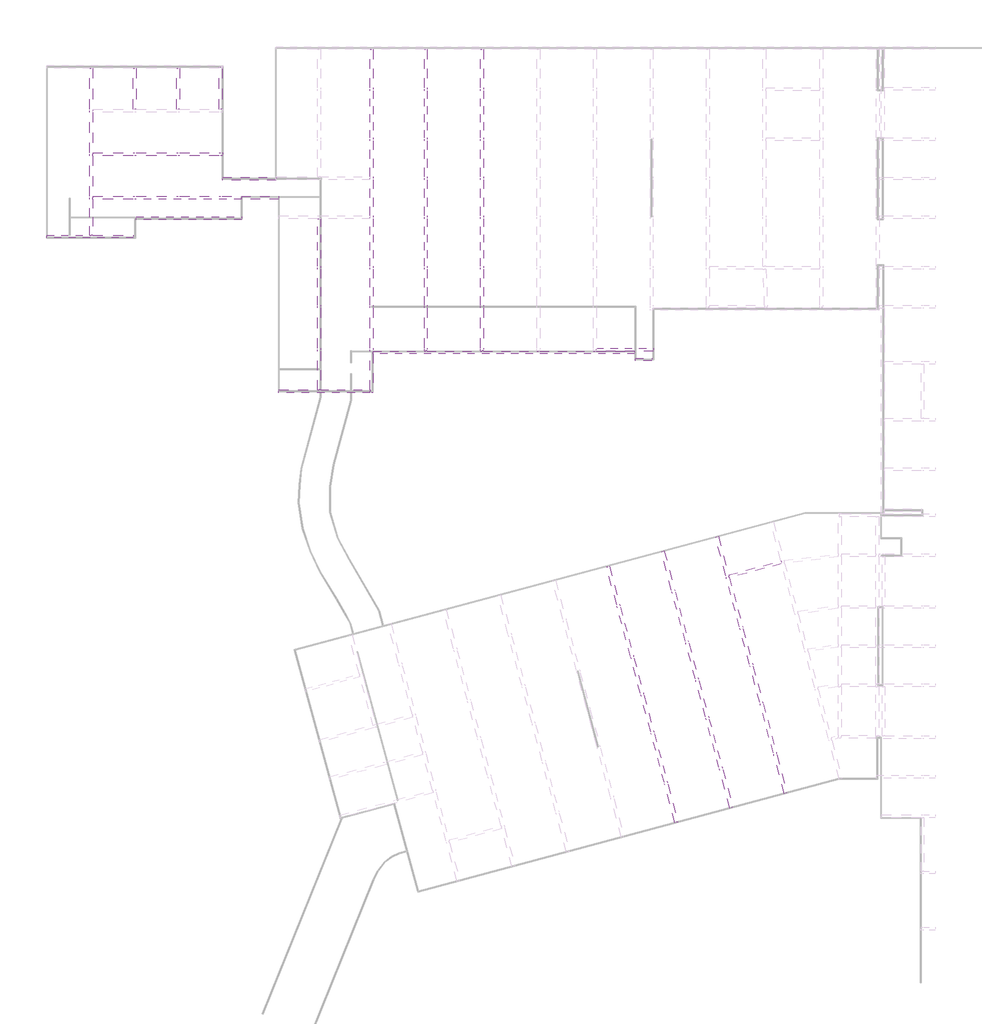
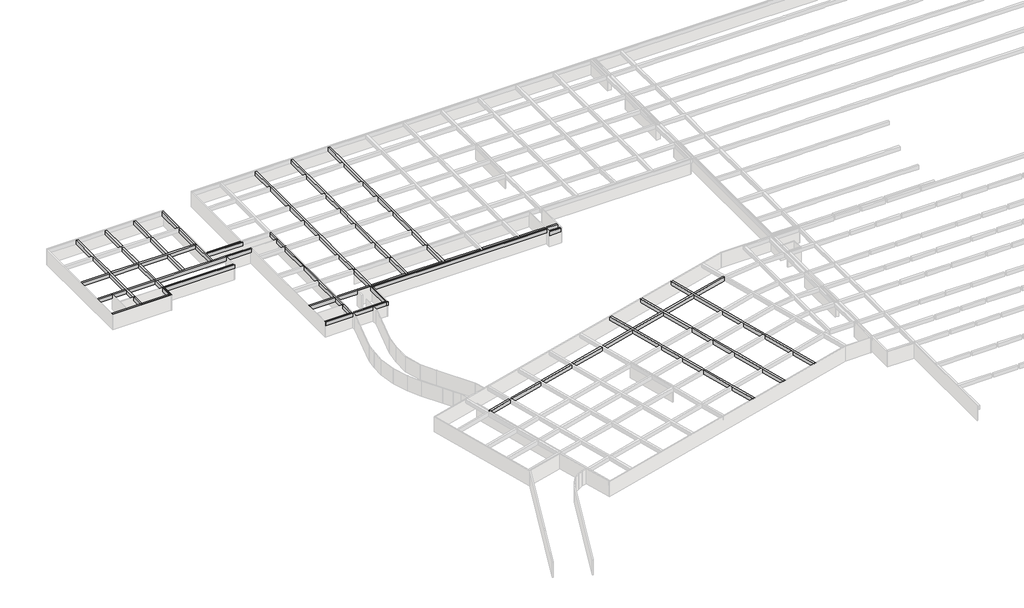
# One storey, part 4 of 14: 22 beams.
"""IFC4 building model written with IfcOpenShell, lengths in millimetres."""

import ifcopenshell
import ifcopenshell.guid

model = None  # the IFC model being written
_history = None  # IfcOwnerHistory: only IFC2X3 demands one
_inside = {}  # id of a spatial element -> (the spatial element, [elements in it])
_under = {}  # id of a project, library or spatial element -> (it, [spatial elements below it])
_declared = {}  # id of a project -> (the project, [libraries it declares])
_typed = {}  # id of a type object -> (the type object, [elements of that type])
_made_of = {}  # id of a material, layer set ... -> (it, [elements and type objects made of it])


def new_model(schema):
    """Start an empty IFC model of exactly this schema.

    Asked for "IFC4X3", IfcOpenShell would pick the latest addendum, in which some entities
    have other attributes; the version numbers below select the first issue.
    IFC2X3 requires an IfcOwnerHistory on every rooted entity: one is made here for all.
    """
    global model, _history
    if schema == "IFC4X3":
        model = ifcopenshell.file(schema_version=(4, 3, 0, 0))
    else:
        model = ifcopenshell.file(schema=schema)
    _inside.clear()
    _under.clear()
    _declared.clear()
    _typed.clear()
    _made_of.clear()
    _history = None
    if model.schema == "IFC2X3":
        org = make("IfcOrganization", Name="unknown")
        user = make(
            "IfcPersonAndOrganization",
            ThePerson=make("IfcPerson", FamilyName="unknown"),
            TheOrganization=org,
        )
        app = make(
            "IfcApplication",
            ApplicationDeveloper=org,
            Version="unknown",
            ApplicationFullName="unknown",
            ApplicationIdentifier="unknown",
        )
        _history = make(
            "IfcOwnerHistory",
            OwningUser=user,
            OwningApplication=app,
            ChangeAction="ADDED",
            CreationDate=0,
        )
    return model


def make(cls, **values):
    """One entity of the class cls with the attributes given. An attribute that is None is left unset."""
    return model.create_entity(
        cls, **{name: value for name, value in values.items() if value is not None}
    )


def rooted(cls, **values):
    """An entity with a GlobalId (a new one), such as an element, a storey or a relation."""
    return make(cls, GlobalId=ifcopenshell.guid.new(), OwnerHistory=_history, **values)


def si_unit(unit_type, name, prefix=None):
    """IfcSIUnit, for example si_unit("LENGTHUNIT", "METRE", prefix="MILLI")."""
    return make("IfcSIUnit", UnitType=unit_type, Prefix=prefix, Name=name)


def assignment(units):
    """IfcUnitAssignment: the units of a project."""
    return None if units is None else make("IfcUnitAssignment", Units=units)


def point(xyz):
    """IfcCartesianPoint."""
    return None if xyz is None else make("IfcCartesianPoint", Coordinates=xyz)


def direction(xyz):
    """IfcDirection."""
    return None if xyz is None else make("IfcDirection", DirectionRatios=xyz)


def frame(location, z_axis=None, x_axis=None):
    """IfcAxis2Placement3D, a coordinate frame: its origin and axes. An axis left out is left unset."""
    return make(
        "IfcAxis2Placement3D",
        Location=point(location),
        Axis=direction(z_axis),
        RefDirection=direction(x_axis),
    )


def origin():
    """The frame at (0, 0, 0) with its axes left unset."""
    return frame((0.0, 0.0, 0.0))


def place(relative_to, where):
    """IfcLocalPlacement: puts the frame where relative to a parent placement (None: the world)."""
    return make(
        "IfcLocalPlacement", PlacementRelTo=relative_to, RelativePlacement=where
    )


def context(
    kind, dimensions, precision=None, world=None, true_north=None, identifier=None
):
    """IfcGeometricRepresentationContext, for example the 3D "Model" context."""
    return make(
        "IfcGeometricRepresentationContext",
        ContextIdentifier=identifier,
        ContextType=kind,
        CoordinateSpaceDimension=dimensions,
        Precision=precision,
        WorldCoordinateSystem=world,
        TrueNorth=true_north,
    )


def project(units=None, contexts=None):
    """IfcProject with its units and contexts."""
    return rooted(
        "IfcProject",
        Name="project",
        RepresentationContexts=contexts,
        UnitsInContext=assignment(units),
    )


def spatial(cls, under=None, at=None, **own):
    """A site, building, storey or space (cls), placed at a placement, below another one or the project."""
    s = rooted(cls, ObjectPlacement=at, **own)
    if under is not None:
        _under.setdefault(under.id(), (under, []))[1].append(s)
    return s


def polyline(points):
    """IfcPolyline through the points."""
    return make("IfcPolyline", Points=[point(p) for p in points])


def outline(outer, holes=None, kind="AREA"):
    """IfcArbitraryClosedProfileDef: a profile drawn as a closed curve; with holes, ...WithVoids."""
    if holes is None:
        return make("IfcArbitraryClosedProfileDef", ProfileType=kind, OuterCurve=outer)
    return make(
        "IfcArbitraryProfileDefWithVoids",
        ProfileType=kind,
        OuterCurve=outer,
        InnerCurves=holes,
    )


def extrude(swept, where, along, depth):
    """IfcExtrudedAreaSolid: the profile swept, set in the frame where, extruded along a direction by depth."""
    return make(
        "IfcExtrudedAreaSolid",
        SweptArea=swept,
        Position=where,
        ExtrudedDirection=direction(along),
        Depth=depth,
    )


def faces_of(points, faces, orient=None, outer=None):
    """IfcFace entities. A face is a list of loops; a loop is a list of indices into points, from 0.

    orient and outer hold one flag for each loop. By default every Orientation is true, the
    first loop of a face is its IfcFaceOuterBound and the others are IfcFaceBound.
    """
    made = []
    for i, loops in enumerate(faces):
        bounds = []
        for j, loop in enumerate(loops):
            is_outer = j == 0 if outer is None else outer[i][j]
            bounds.append(
                make(
                    "IfcFaceOuterBound" if is_outer else "IfcFaceBound",
                    Bound=make("IfcPolyLoop", Polygon=[points[k] for k in loop]),
                    Orientation=True if orient is None else orient[i][j],
                )
            )
        made.append(make("IfcFace", Bounds=bounds))
    return made


def faceted_brep(points, faces, orient=None, outer=None, voids=None):
    """IfcFacetedBrep: a solid bounded by flat faces; with voids (closed shells), ...WithVoids."""
    shared = [point(p) for p in points]
    hull = make("IfcClosedShell", CfsFaces=faces_of(shared, faces, orient, outer))
    if voids is None:
        return make("IfcFacetedBrep", Outer=hull)
    return make(
        "IfcFacetedBrepWithVoids",
        Outer=hull,
        Voids=[
            make(cls, CfsFaces=faces_of(shared, fs, o, b)) for cls, fs, o, b in voids
        ],
    )


def shape(context_of_items, identifier, shape_type, items):
    """IfcShapeRepresentation: the items that make up one representation, for example the "Body"."""
    return make(
        "IfcShapeRepresentation",
        ContextOfItems=context_of_items,
        RepresentationIdentifier=identifier,
        RepresentationType=shape_type,
        Items=items,
    )


def source(mapping_origin, context_of_items, identifier, shape_type, items):
    """IfcRepresentationMap: a shape defined once, which mapped items show again and again."""
    return make(
        "IfcRepresentationMap",
        MappingOrigin=mapping_origin,
        MappedRepresentation=shape(context_of_items, identifier, shape_type, items),
    )


def transform(
    local_origin,
    x_axis=None,
    y_axis=None,
    z_axis=None,
    scale=None,
    scale2=None,
    scale3=None,
    uniform=True,
):
    """IfcCartesianTransformationOperator3D, or its non-uniform kind. x_axis, y_axis, z_axis: its Axis1, 2, 3."""
    if uniform:
        return make(
            "IfcCartesianTransformationOperator3D",
            Axis1=direction(x_axis),
            Axis2=direction(y_axis),
            LocalOrigin=point(local_origin),
            Scale=scale,
            Axis3=direction(z_axis),
        )
    return make(
        "IfcCartesianTransformationOperator3DnonUniform",
        Axis1=direction(x_axis),
        Axis2=direction(y_axis),
        LocalOrigin=point(local_origin),
        Scale=scale,
        Axis3=direction(z_axis),
        Scale2=scale2,
        Scale3=scale3,
    )


def mapped(mapping_source, mapping_target):
    """IfcMappedItem: shows the shape of a source again, moved by a transform."""
    return make(
        "IfcMappedItem", MappingSource=mapping_source, MappingTarget=mapping_target
    )


def made_of(thing, what):
    """Note that an element or type object is made of a material, layer set ...; save() writes the relation."""
    if what is not None:
        _made_of.setdefault(what.id(), (what, []))[1].append(thing)
    return thing


def element(
    cls,
    number,
    at=None,
    inside=None,
    cuts=None,
    type_object=None,
    material=None,
    context=None,
    identifier="Body",
    shape_type=None,
    held_by="IfcProductDefinitionShape",
    body=None,
    shapes=None,
    **own,
):
    """One element of the class cls, such as IfcWall. Its Tag is "e" and its number.

    at: its placement. inside: the storey or other place that contains it. cuts: it is an
    opening in that element (IfcRelVoidsElement). A single representation is given by context,
    identifier, shape_type and body (its items); several are given by shapes. held_by: the class
    of the entity that holds the representations. save() writes the other relations.
    """
    e = rooted(cls, Tag="e%d" % number, ObjectPlacement=at, **own)
    if body is not None:
        shapes = [shape(context, identifier, shape_type, body)]
    if shapes is not None:
        e.Representation = make(held_by, Representations=shapes)
    if inside is not None:
        _inside.setdefault(inside.id(), (inside, []))[1].append(e)
    if cuts is not None:
        rooted(
            "IfcRelVoidsElement", RelatingBuildingElement=cuts, RelatedOpeningElement=e
        )
    if type_object is not None:
        _typed.setdefault(type_object.id(), (type_object, []))[1].append(e)
    return made_of(e, material)


def aggregate(whole, parts):
    """IfcRelAggregates: a whole, such as a stair, and the parts it consists of."""
    return rooted("IfcRelAggregates", RelatingObject=whole, RelatedObjects=parts)


def save(model, path):
    """Write the relations noted so far, then the file.

    IfcRelAggregates (storeys below a building ...), IfcRelContainedInSpatialStructure (elements
    in a storey), IfcRelDefinesByType, IfcRelAssociatesMaterial and IfcRelDeclares: one each for
    every whole, place, type object, material and project.
    """
    for whole, parts in _under.values():
        aggregate(whole, parts)
    for where, things in _inside.values():
        rooted(
            "IfcRelContainedInSpatialStructure",
            RelatedElements=things,
            RelatingStructure=where,
        )
    for kind, things in _typed.values():
        rooted("IfcRelDefinesByType", RelatedObjects=things, RelatingType=kind)
    for what, things in _made_of.values():
        rooted("IfcRelAssociatesMaterial", RelatedObjects=things, RelatingMaterial=what)
    for by, libraries in _declared.values():
        rooted("IfcRelDeclares", RelatingContext=by, RelatedDefinitions=libraries)
    model.write(path)


def kl_beam_2b0aae00(model_context):
    return source(origin(), model_context, "Body", "SweptSolid", [
        extrude(outline(polyline([(1133.5, 200.0), (1133.5, -200.0), (-1133.5, -200.0), (-1133.5, 200.0), (1133.5, 200.0)])), frame((0.0, 0.0, -400.0), z_axis=(0.0, 0.0, 1.0), x_axis=(1.0, 0.0, 0.0)), (0.0, 0.0, 1.0), 800.0),
    ])


model = new_model("IFC4")

# Units and contexts
model_context = context("Model", 3, world=origin())
ifc_project = project(units=[si_unit("LENGTHUNIT", "METRE", prefix="MILLI")], contexts=[model_context])

# Site, building, storey
site = spatial("IfcSite", under=ifc_project)
building = spatial("IfcBuilding", under=site)
storey = spatial("IfcBuildingStorey", under=building, Name="户型图", Elevation=0.0)

# Beams
placement = place(None, origin())
element("IfcBeam", 1, ObjectType="混凝土 - 矩形梁 : KL_beam", at=placement, inside=storey, context=model_context, shape_type="Brep", body=[
    faceted_brep([(-96064.0025134, -143183.950757, 3300.0), (-95664.0025134, -143183.950757, 3300.0), (-95664.0025134, -138262.0857972, 3300.0), (-95664.0025134, -137862.0857972, 3300.0), (-95664.0025134, -132244.4272419, 3300.0), (-95664.0025134, -131844.4272419, 3300.0), (-95664.0025134, -126236.5894684, 3300.0), (-95664.0025134, -125836.5894684, 3300.0), (-95664.0025134, -120134.1750557, 3300.0), (-96064.0025134, -120134.1750557, 3300.0), (-96064.0025134, -125836.5894684, 3300.0), (-96064.0025134, -126236.5894684, 3300.0), (-96064.0025134, -131844.4272419, 3300.0), (-96064.0025134, -132244.4272419, 3300.0), (-96064.0025134, -137862.0857972, 3300.0), (-96064.0025134, -138262.0857972, 3300.0), (-96064.0025134, -143183.950757, 2500.0), (-96064.0025134, -120134.1750557, 2500.0), (-96064.0025134, -125836.5894684, 2500.0), (-96064.0025134, -126236.5894684, 2500.0), (-96064.0025134, -131844.4272419, 2500.0), (-96064.0025134, -132244.4272419, 2500.0), (-96064.0025134, -137862.0857972, 2500.0), (-96064.0025134, -138262.0857972, 2500.0), (-95664.0025134, -143183.950757, 2500.0), (-95664.0025134, -120134.1750557, 2500.0), (-95664.0025134, -125836.5894684, 2500.0), (-95664.0025134, -126236.5894684, 2500.0), (-95664.0025134, -131844.4272419, 2500.0), (-95664.0025134, -132244.4272419, 2500.0), (-95664.0025134, -137862.0857972, 2500.0), (-95664.0025134, -138262.0857972, 2500.0)], [[[0, 1, 2, 3, 4, 5, 6, 7, 8, 9, 10, 11, 12, 13, 14, 15]], [[16, 0, 15, 14, 13, 12, 11, 10, 9, 17, 18, 19, 20, 21, 22, 23]], [[24, 16, 23, 22, 21, 20, 19, 18, 17, 25, 26, 27, 28, 29, 30, 31]], [[1, 24, 31, 30, 29, 28, 27, 26, 25, 8, 7, 6, 5, 4, 3, 2]], [[1, 0, 16, 24]], [[9, 8, 25, 17]]]),
])
element("IfcBeam", 2, ObjectType="混凝土 - 矩形梁 : KL_beam", at=placement, inside=storey, context=model_context, shape_type="Brep", body=[
    faceted_brep([(-77750.8485237, -131844.4272419, 3300.0), (-77750.8485237, -132244.4272419, 3300.0), (-77750.8485237, -132244.4272419, 2500.0), (-77750.8485237, -131844.4272419, 2500.0), (-77800.8485237, -131844.4272419, 3300.0), (-78200.8485237, -131844.4272419, 3300.0), (-83675.8485237, -131844.4272419, 3300.0), (-84075.8485237, -131844.4272419, 3300.0), (-89675.8485237, -131844.4272419, 3300.0), (-90075.8485237, -131844.4272419, 3300.0), (-95664.0025134, -131844.4272419, 3300.0), (-95664.0025134, -132244.4272419, 3300.0), (-90075.8485237, -132244.4272419, 3300.0), (-89675.8485237, -132244.4272419, 3300.0), (-84075.8485237, -132244.4272419, 3300.0), (-83675.8485237, -132244.4272419, 3300.0), (-78200.8485237, -132244.4272419, 3300.0), (-77800.8485237, -132244.4272419, 3300.0), (-95664.0025134, -132244.4272419, 2500.0), (-90075.8485237, -132244.4272419, 2500.0), (-89675.8485237, -132244.4272419, 2500.0), (-84075.8485237, -132244.4272419, 2500.0), (-83675.8485237, -132244.4272419, 2500.0), (-78200.8485237, -132244.4272419, 2500.0), (-77800.8485237, -132244.4272419, 2500.0), (-95664.0025134, -131844.4272419, 2500.0), (-90075.8485237, -131844.4272419, 2500.0), (-89675.8485237, -131844.4272419, 2500.0), (-84075.8485237, -131844.4272419, 2500.0), (-83675.8485237, -131844.4272419, 2500.0), (-78200.8485237, -131844.4272419, 2500.0), (-77800.8485237, -131844.4272419, 2500.0)], [[[0, 1, 2, 3]], [[1, 0, 4, 5, 6, 7, 8, 9, 10, 11, 12, 13, 14, 15, 16, 17]], [[2, 1, 17, 16, 15, 14, 13, 12, 11, 18, 19, 20, 21, 22, 23, 24]], [[3, 2, 24, 23, 22, 21, 20, 19, 18, 25, 26, 27, 28, 29, 30, 31]], [[0, 3, 31, 30, 29, 28, 27, 26, 25, 10, 9, 8, 7, 6, 5, 4]], [[11, 10, 25, 18]]]),
    faceted_brep([(-102000.8485237, -131844.4272419, 3300.0), (-102000.8485237, -131844.4272419, 2500.0), (-102000.8485237, -132244.4272419, 2500.0), (-102000.8485237, -132244.4272419, 3300.0), (-96064.0025134, -131844.4272419, 3300.0), (-96064.0025134, -132244.4272419, 3300.0), (-96064.0025134, -132244.4272419, 2500.0), (-96064.0025134, -131844.4272419, 2500.0)], [[[0, 1, 2, 3]], [[4, 5, 6, 7]], [[0, 3, 5, 4]], [[3, 2, 6, 5]], [[2, 1, 7, 6]], [[1, 0, 4, 7]]]),
])
element("IfcBeam", 3, ObjectType="混凝土 - 矩形梁 : KL_beam", at=placement, inside=storey, context=model_context, shape_type="Brep", body=[
    faceted_brep([(-102000.8485237, -137862.0857972, 3300.0), (-102000.8485237, -137862.0857972, 2500.0), (-102000.8485237, -138262.0857972, 2500.0), (-102000.8485237, -138262.0857972, 3300.0), (-96064.0025134, -137862.0857972, 3300.0), (-96064.0025134, -138262.0857972, 3300.0), (-96064.0025134, -138262.0857972, 2500.0), (-96064.0025134, -137862.0857972, 2500.0)], [[[0, 1, 2, 3]], [[4, 5, 6, 7]], [[0, 3, 5, 4]], [[3, 2, 6, 5]], [[2, 1, 7, 6]], [[1, 0, 4, 7]]]),
    faceted_brep([(-75125.8485237, -138262.0857972, 3300.0), (-75125.8485237, -137862.0857972, 3300.0), (-77800.8485237, -137862.0857972, 3300.0), (-78200.8485237, -137862.0857972, 3300.0), (-83675.8485237, -137862.0857972, 3300.0), (-84075.8485237, -137862.0857972, 3300.0), (-89675.8485237, -137862.0857972, 3300.0), (-90075.8485237, -137862.0857972, 3300.0), (-95664.0025134, -137862.0857972, 3300.0), (-95664.0025134, -138262.0857972, 3300.0), (-90075.8485237, -138262.0857972, 3300.0), (-89675.8485237, -138262.0857972, 3300.0), (-75125.8485237, -138262.0857972, 2500.0), (-95664.0025134, -138262.0857972, 2500.0), (-90075.8485237, -138262.0857972, 2500.0), (-89675.8485237, -138262.0857972, 2500.0), (-75125.8485237, -137862.0857972, 2500.0), (-95664.0025134, -137862.0857972, 2500.0), (-90075.8485237, -137862.0857972, 2500.0), (-89675.8485237, -137862.0857972, 2500.0), (-84075.8485237, -137862.0857972, 2500.0), (-83675.8485237, -137862.0857972, 2500.0), (-78200.8485237, -137862.0857972, 2500.0), (-77800.8485237, -137862.0857972, 2500.0)], [[[0, 1, 2, 3, 4, 5, 6, 7, 8, 9, 10, 11]], [[12, 0, 11, 10, 9, 13, 14, 15]], [[16, 12, 15, 14, 13, 17, 18, 19, 20, 21, 22, 23]], [[1, 16, 23, 22, 21, 20, 19, 18, 17, 8, 7, 6, 5, 4, 3, 2]], [[9, 8, 17, 13]], [[1, 0, 12, 16]]]),
])
element("IfcBeam", 4, ObjectType="混凝土 - 矩形梁 : KL_beam", at=placement, inside=storey, context=model_context, shape_type="Brep", body=[
    faceted_brep([(-90075.8485237, -125836.5894684, 3300.0), (-89675.8485237, -125836.5894684, 3300.0), (-89675.8485237, -120134.1750557, 3300.0), (-90075.8485237, -120134.1750557, 3300.0), (-90075.8485237, -125836.5894684, 2500.0), (-90075.8485237, -120134.1750557, 2500.0), (-89675.8485237, -125836.5894684, 2500.0), (-89675.8485237, -120134.1750557, 2500.0)], [[[0, 1, 2, 3]], [[4, 0, 3, 5]], [[6, 4, 5, 7]], [[1, 6, 7, 2]], [[1, 0, 4, 6]], [[3, 2, 7, 5]]]),
    faceted_brep([(-90075.8485237, -126236.5894684, 3300.0), (-89675.8485237, -126236.5894684, 3300.0), (-89675.8485237, -126236.5894684, 2500.0), (-90075.8485237, -126236.5894684, 2500.0), (-89675.8485237, -131844.4272419, 3300.0), (-90075.8485237, -131844.4272419, 3300.0), (-90075.8485237, -131844.4272419, 2500.0), (-89675.8485237, -131844.4272419, 2500.0)], [[[0, 1, 2, 3]], [[4, 5, 6, 7]], [[1, 0, 5, 4]], [[0, 3, 6, 5]], [[3, 2, 7, 6]], [[2, 1, 4, 7]]]),
    faceted_brep([(-89675.8485237, -132244.4272419, 3300.0), (-90075.8485237, -132244.4272419, 3300.0), (-90075.8485237, -137862.0857972, 3300.0), (-89675.8485237, -137862.0857972, 3300.0), (-90075.8485237, -132244.4272419, 2500.0), (-90075.8485237, -137862.0857972, 2500.0), (-89675.8485237, -132244.4272419, 2500.0), (-89675.8485237, -137862.0857972, 2500.0)], [[[0, 1, 2, 3]], [[1, 4, 5, 2]], [[4, 6, 7, 5]], [[6, 0, 3, 7]], [[1, 0, 6, 4]], [[3, 2, 5, 7]]]),
    faceted_brep([(-90075.8485237, -138262.0857972, 3300.0), (-89675.8485237, -138262.0857972, 3300.0), (-89675.8485237, -138262.0857972, 2500.0), (-90075.8485237, -138262.0857972, 2500.0), (-89675.8485237, -143583.950757, 3300.0), (-90075.8485237, -143583.950757, 3300.0), (-90075.8485237, -143583.950757, 2500.0), (-89675.8485237, -143583.950757, 2500.0), (-89675.8485237, -141083.950757, 3300.0), (-89675.8485237, -140683.950757, 3300.0), (-90075.8485237, -143183.950757, 3300.0), (-90075.8485237, -143183.950757, 2500.0), (-89675.8485237, -140683.950757, 2500.0), (-89675.8485237, -141083.950757, 2500.0)], [[[0, 1, 2, 3]], [[4, 5, 6, 7]], [[5, 4, 8, 9, 1, 0, 10]], [[6, 5, 10, 0, 3, 11]], [[7, 6, 11, 3, 2, 12, 13]], [[4, 7, 13, 12, 2, 1, 9, 8]]]),
])
element("IfcBeam", 5, ObjectType="混凝土 - 矩形梁 : KL_beam", at=placement, inside=storey, context=model_context, shape_type="SweptSolid", body=[
    extrude(outline(polyline([(-83675.8485237, -125836.5894684), (-84075.8485237, -125836.5894684), (-84075.8485237, -120134.1750557), (-83675.8485237, -120134.1750557), (-83675.8485237, -125836.5894684)])), frame((0.0, 0.0, 2500.0), z_axis=(0.0, 0.0, 1.0), x_axis=(1.0, 0.0, 0.0)), (0.0, 0.0, 1.0), 800.0),
    extrude(outline(polyline([(-83675.8485237, -137862.0857972), (-84075.8485237, -137862.0857972), (-84075.8485237, -132244.4272419), (-83675.8485237, -132244.4272419), (-83675.8485237, -137862.0857972)])), frame((0.0, 0.0, 2500.0), z_axis=(0.0, 0.0, 1.0), x_axis=(1.0, 0.0, 0.0)), (0.0, 0.0, 1.0), 800.0),
    extrude(outline(polyline([(-84075.8485237, -126236.5894684), (-83675.8485237, -126236.5894684), (-83675.8485237, -131844.4272419), (-84075.8485237, -131844.4272419), (-84075.8485237, -126236.5894684)])), frame((0.0, 0.0, 2500.0), z_axis=(0.0, 0.0, 1.0), x_axis=(1.0, 0.0, 0.0)), (0.0, 0.0, 1.0), 800.0),
])
element("IfcBeam", 6, ObjectType="混凝土 - 矩形梁 : KL_beam", at=placement, inside=storey, context=model_context, shape_type="Brep", body=[
    faceted_brep([(-78200.8485237, -119934.6304265, 3300.0), (-77800.8485237, -119934.6304265, 3300.0), (-77800.8485237, -119934.6304265, 2500.0), (-78200.8485237, -119934.6304265, 2500.0), (-78200.8485237, -120134.1750557, 3300.0), (-78200.8485237, -125836.5894684, 3300.0), (-77800.8485237, -125836.5894684, 3300.0), (-77800.8485237, -120134.1750557, 3300.0), (-77800.8485237, -125836.5894684, 2500.0), (-77800.8485237, -120134.1750557, 2500.0), (-78200.8485237, -125836.5894684, 2500.0), (-78200.8485237, -120134.1750557, 2500.0)], [[[0, 1, 2, 3]], [[1, 0, 4, 5, 6, 7]], [[2, 1, 7, 6, 8, 9]], [[3, 2, 9, 8, 10, 11]], [[0, 3, 11, 10, 5, 4]], [[6, 5, 10, 8]]]),
    faceted_brep([(-77800.8485237, -137862.0857972, 3300.0), (-78200.8485237, -137862.0857972, 3300.0), (-78200.8485237, -137862.0857972, 2500.0), (-77800.8485237, -137862.0857972, 2500.0), (-78200.8485237, -132244.4272419, 3300.0), (-77800.8485237, -132244.4272419, 3300.0), (-77800.8485237, -132244.4272419, 2500.0), (-78200.8485237, -132244.4272419, 2500.0)], [[[0, 1, 2, 3]], [[4, 5, 6, 7]], [[1, 0, 5, 4]], [[0, 3, 6, 5]], [[3, 2, 7, 6]], [[2, 1, 4, 7]]]),
    faceted_brep([(-78200.8485237, -126236.5894684, 3300.0), (-77800.8485237, -126236.5894684, 3300.0), (-77800.8485237, -126236.5894684, 2500.0), (-78200.8485237, -126236.5894684, 2500.0), (-78200.8485237, -131844.4272419, 3300.0), (-77800.8485237, -131844.4272419, 3300.0), (-77800.8485237, -131844.4272419, 2500.0), (-78200.8485237, -131844.4272419, 2500.0)], [[[0, 1, 2, 3]], [[1, 0, 4, 5]], [[2, 1, 5, 6]], [[3, 2, 6, 7]], [[0, 3, 7, 4]], [[5, 4, 7, 6]]]),
])
element("IfcBeam", 7, ObjectType="混凝土 - 矩形梁 : KL_beam", at=placement, inside=storey, context=model_context, shape_type="Brep", body=[
    faceted_brep([(-57355.3281677, -164958.1892784, 3300.0), (-56955.3281677, -164958.1892784, 3300.0), (-56955.3281677, -159558.4277999, 3300.0), (-56955.3281677, -159207.3751505, 3300.0), (-56955.3281677, -158807.3751505, 3300.0), (-56955.3281677, -153248.950757, 3300.0), (-56955.3281677, -152848.950757, 3300.0), (-56955.3281677, -147899.284307, 3300.0), (-56955.3281677, -147499.284307, 3300.0), (-56955.3281677, -140920.0179086, 3300.0), (-56955.3281677, -140520.0179086, 3300.0), (-56955.3281677, -135526.4975491, 3300.0), (-56955.3281677, -135126.4975491, 3300.0), (-56955.3281677, -130180.0179086, 3300.0), (-56955.3281677, -129780.0179086, 3300.0), (-56955.3281677, -123258.950757, 3300.0), (-56955.3281677, -122858.950757, 3300.0), (-56955.3281677, -117558.950757, 3300.0), (-57355.3281677, -117558.950757, 3300.0), (-57355.3281677, -122858.950757, 3300.0), (-57355.3281677, -123258.950757, 3300.0), (-57355.3281677, -129780.0179086, 3300.0), (-57355.3281677, -130180.0179086, 3300.0), (-57355.3281677, -135126.4975491, 3300.0), (-57355.3281677, -135526.4975491, 3300.0), (-57355.3281677, -140520.0179086, 3300.0), (-57355.3281677, -140920.0179086, 3300.0), (-57355.3281677, -147499.284307, 3300.0), (-57355.3281677, -147899.284307, 3300.0), (-57355.3281677, -152848.950757, 3300.0), (-57355.3281677, -153248.950757, 3300.0), (-57355.3281677, -158807.3751505, 3300.0), (-57355.3281677, -159207.3751505, 3300.0), (-57355.3281677, -164558.1892784, 3300.0), (-57355.3281677, -164958.1892784, 2500.0), (-57355.3281677, -117558.950757, 2500.0), (-57355.3281677, -122858.950757, 2500.0), (-57355.3281677, -123258.950757, 2500.0), (-57355.3281677, -129780.0179086, 2500.0), (-57355.3281677, -130180.0179086, 2500.0), (-57355.3281677, -135126.4975491, 2500.0), (-57355.3281677, -135526.4975491, 2500.0), (-57355.3281677, -140520.0179086, 2500.0), (-57355.3281677, -140920.0179086, 2500.0), (-57355.3281677, -147499.284307, 2500.0), (-57355.3281677, -147899.284307, 2500.0), (-57355.3281677, -152848.950757, 2500.0), (-57355.3281677, -153248.950757, 2500.0), (-57355.3281677, -158807.3751505, 2500.0), (-57355.3281677, -159207.3751505, 2500.0), (-57355.3281677, -164558.1892784, 2500.0), (-56955.3281677, -164958.1892784, 2500.0), (-56955.3281677, -117558.950757, 2500.0), (-56955.3281677, -122858.950757, 2500.0), (-56955.3281677, -123258.950757, 2500.0), (-56955.3281677, -129780.0179086, 2500.0), (-56955.3281677, -130180.0179086, 2500.0), (-56955.3281677, -135126.4975491, 2500.0), (-56955.3281677, -135526.4975491, 2500.0), (-56955.3281677, -140520.0179086, 2500.0), (-56955.3281677, -140920.0179086, 2500.0), (-56955.3281677, -147499.284307, 2500.0), (-56955.3281677, -147899.284307, 2500.0), (-56955.3281677, -152848.950757, 2500.0), (-56955.3281677, -153248.950757, 2500.0), (-56955.3281677, -158807.3751505, 2500.0), (-56955.3281677, -159207.3751505, 2500.0), (-56955.3281677, -159558.4277999, 2500.0)], [[[0, 1, 2, 3, 4, 5, 6, 7, 8, 9, 10, 11, 12, 13, 14, 15, 16, 17, 18, 19, 20, 21, 22, 23, 24, 25, 26, 27, 28, 29, 30, 31, 32, 33]], [[34, 0, 33, 32, 31, 30, 29, 28, 27, 26, 25, 24, 23, 22, 21, 20, 19, 18, 35, 36, 37, 38, 39, 40, 41, 42, 43, 44, 45, 46, 47, 48, 49, 50]], [[51, 34, 50, 49, 48, 47, 46, 45, 44, 43, 42, 41, 40, 39, 38, 37, 36, 35, 52, 53, 54, 55, 56, 57, 58, 59, 60, 61, 62, 63, 64, 65, 66, 67]], [[1, 51, 67, 66, 65, 64, 63, 62, 61, 60, 59, 58, 57, 56, 55, 54, 53, 52, 17, 16, 15, 14, 13, 12, 11, 10, 9, 8, 7, 6, 5, 4, 3, 2]], [[1, 0, 34, 51]], [[18, 17, 52, 35]]]),
])
element("IfcBeam", 8, ObjectType="混凝土 - 矩形梁 : KL_beam", at=placement, inside=storey, context=model_context, shape_type="Brep", body=[
    faceted_brep([(-49869.9201432, -159158.4277999, 3300.0), (-49469.9201432, -159158.4277999, 3300.0), (-49469.9201432, -158807.3751505, 3300.0), (-49469.9201432, -153248.950757, 3300.0), (-49469.9201432, -152848.950757, 3300.0), (-49469.9201432, -147899.284307, 3300.0), (-49469.9201432, -147499.284307, 3300.0), (-49469.9201432, -140920.0179086, 3300.0), (-49469.9201432, -140520.0179086, 3300.0), (-49469.9201432, -135526.4975491, 3300.0), (-49469.9201432, -135126.4975491, 3300.0), (-49469.9201432, -130180.0179086, 3300.0), (-49469.9201432, -129780.0179086, 3300.0), (-49469.9201432, -123258.950757, 3300.0), (-49469.9201432, -122858.950757, 3300.0), (-49469.9201432, -117558.950757, 3300.0), (-49869.9201432, -117558.950757, 3300.0), (-49869.9201432, -122858.950757, 3300.0), (-49869.9201432, -123258.950757, 3300.0), (-49869.9201432, -129780.0179086, 3300.0), (-49869.9201432, -130180.0179086, 3300.0), (-49869.9201432, -135126.4975491, 3300.0), (-49869.9201432, -135526.4975491, 3300.0), (-49869.9201432, -140520.0179086, 3300.0), (-49869.9201432, -140920.0179086, 3300.0), (-49869.9201432, -147499.284307, 3300.0), (-49869.9201432, -147899.284307, 3300.0), (-49869.9201432, -152848.950757, 3300.0), (-49869.9201432, -153248.950757, 3300.0), (-49869.9201432, -158807.3751505, 3300.0), (-49869.9201432, -159158.4277999, 2500.0), (-49869.9201432, -117558.950757, 2500.0), (-49869.9201432, -122858.950757, 2500.0), (-49869.9201432, -123258.950757, 2500.0), (-49869.9201432, -129780.0179086, 2500.0), (-49869.9201432, -130180.0179086, 2500.0), (-49869.9201432, -135126.4975491, 2500.0), (-49869.9201432, -135526.4975491, 2500.0), (-49869.9201432, -140520.0179086, 2500.0), (-49869.9201432, -140920.0179086, 2500.0), (-49869.9201432, -147499.284307, 2500.0), (-49869.9201432, -147899.284307, 2500.0), (-49869.9201432, -152848.950757, 2500.0), (-49869.9201432, -153248.950757, 2500.0), (-49869.9201432, -158807.3751505, 2500.0), (-49469.9201432, -159158.4277999, 2500.0), (-49469.9201432, -117558.950757, 2500.0), (-49469.9201432, -122858.950757, 2500.0), (-49469.9201432, -123258.950757, 2500.0), (-49469.9201432, -129780.0179086, 2500.0), (-49469.9201432, -130180.0179086, 2500.0), (-49469.9201432, -135126.4975491, 2500.0), (-49469.9201432, -135526.4975491, 2500.0), (-49469.9201432, -140520.0179086, 2500.0), (-49469.9201432, -140920.0179086, 2500.0), (-49469.9201432, -147499.284307, 2500.0), (-49469.9201432, -147899.284307, 2500.0), (-49469.9201432, -152848.950757, 2500.0), (-49469.9201432, -153248.950757, 2500.0), (-49469.9201432, -158807.3751505, 2500.0)], [[[0, 1, 2, 3, 4, 5, 6, 7, 8, 9, 10, 11, 12, 13, 14, 15, 16, 17, 18, 19, 20, 21, 22, 23, 24, 25, 26, 27, 28, 29]], [[30, 0, 29, 28, 27, 26, 25, 24, 23, 22, 21, 20, 19, 18, 17, 16, 31, 32, 33, 34, 35, 36, 37, 38, 39, 40, 41, 42, 43, 44]], [[45, 30, 44, 43, 42, 41, 40, 39, 38, 37, 36, 35, 34, 33, 32, 31, 46, 47, 48, 49, 50, 51, 52, 53, 54, 55, 56, 57, 58, 59]], [[1, 45, 59, 58, 57, 56, 55, 54, 53, 52, 51, 50, 49, 48, 47, 46, 15, 14, 13, 12, 11, 10, 9, 8, 7, 6, 5, 4, 3, 2]], [[1, 0, 30, 45]], [[16, 15, 46, 31]]]),
])
element("IfcBeam", 9, ObjectType="混凝土 - 矩形梁 : KL_beam", at=placement, inside=storey, context=model_context, shape_type="Brep", body=[
    faceted_brep([(-42115.0194088, -159158.4277999, 3300.0), (-41715.0194088, -159158.4277999, 3300.0), (-41715.0194088, -158807.3751505, 3300.0), (-41715.0194088, -153248.950757, 3300.0), (-41715.0194088, -152848.950757, 3300.0), (-41715.0194088, -147899.284307, 3300.0), (-41715.0194088, -147499.284307, 3300.0), (-41715.0194088, -140920.0179086, 3300.0), (-41715.0194088, -140520.0179086, 3300.0), (-41715.0194088, -135526.4975491, 3300.0), (-41715.0194088, -135126.4975491, 3300.0), (-41715.0194088, -130180.0179086, 3300.0), (-41715.0194088, -129780.0179086, 3300.0), (-41715.0194088, -123258.950757, 3300.0), (-41715.0194088, -122858.950757, 3300.0), (-41715.0194088, -117558.950757, 3300.0), (-42115.0194088, -117558.950757, 3300.0), (-42115.0194088, -122858.950757, 3300.0), (-42115.0194088, -123258.950757, 3300.0), (-42115.0194088, -129780.0179086, 3300.0), (-42115.0194088, -130180.0179086, 3300.0), (-42115.0194088, -135126.4975491, 3300.0), (-42115.0194088, -135526.4975491, 3300.0), (-42115.0194088, -140520.0179086, 3300.0), (-42115.0194088, -140920.0179086, 3300.0), (-42115.0194088, -147499.284307, 3300.0), (-42115.0194088, -147899.284307, 3300.0), (-42115.0194088, -152848.950757, 3300.0), (-42115.0194088, -153248.950757, 3300.0), (-42115.0194088, -158807.3751505, 3300.0), (-41715.0194088, -159158.4277999, 2500.0), (-41715.0194088, -158807.3751505, 2500.0), (-41715.0194088, -153248.950757, 2500.0), (-41715.0194088, -152848.950757, 2500.0), (-41715.0194088, -147899.284307, 2500.0), (-41715.0194088, -147499.284307, 2500.0), (-41715.0194088, -140920.0179086, 2500.0), (-41715.0194088, -140520.0179086, 2500.0), (-41715.0194088, -135526.4975491, 2500.0), (-41715.0194088, -135126.4975491, 2500.0), (-41715.0194088, -130180.0179086, 2500.0), (-41715.0194088, -129780.0179086, 2500.0), (-41715.0194088, -123258.950757, 2500.0), (-41715.0194088, -122858.950757, 2500.0), (-41715.0194088, -117558.950757, 2500.0), (-42115.0194088, -159158.4277999, 2500.0), (-42115.0194088, -158807.3751505, 2500.0), (-42115.0194088, -153248.950757, 2500.0), (-42115.0194088, -152848.950757, 2500.0), (-42115.0194088, -147899.284307, 2500.0), (-42115.0194088, -147499.284307, 2500.0), (-42115.0194088, -140920.0179086, 2500.0), (-42115.0194088, -140520.0179086, 2500.0), (-42115.0194088, -135526.4975491, 2500.0), (-42115.0194088, -135126.4975491, 2500.0), (-42115.0194088, -130180.0179086, 2500.0), (-42115.0194088, -129780.0179086, 2500.0), (-42115.0194088, -123258.950757, 2500.0), (-42115.0194088, -122858.950757, 2500.0), (-42115.0194088, -117558.950757, 2500.0)], [[[0, 1, 2, 3, 4, 5, 6, 7, 8, 9, 10, 11, 12, 13, 14, 15, 16, 17, 18, 19, 20, 21, 22, 23, 24, 25, 26, 27, 28, 29]], [[1, 30, 31, 32, 33, 34, 35, 36, 37, 38, 39, 40, 41, 42, 43, 44, 15, 14, 13, 12, 11, 10, 9, 8, 7, 6, 5, 4, 3, 2]], [[30, 45, 46, 47, 48, 49, 50, 51, 52, 53, 54, 55, 56, 57, 58, 59, 44, 43, 42, 41, 40, 39, 38, 37, 36, 35, 34, 33, 32, 31]], [[45, 0, 29, 28, 27, 26, 25, 24, 23, 22, 21, 20, 19, 18, 17, 16, 59, 58, 57, 56, 55, 54, 53, 52, 51, 50, 49, 48, 47, 46]], [[1, 0, 45, 30]], [[16, 15, 44, 59]]]),
])
element("IfcBeam", 10, ObjectType="混凝土 - 矩形梁 : KL_beam", at=placement, inside=storey, context=model_context, shape_type="Brep", body=[
    faceted_brep([(-64212.7050956, -135526.4975491, 3300.0), (-64612.7050956, -135526.4975491, 3300.0), (-64612.7050956, -140520.0179086, 3300.0), (-64212.7050956, -140520.0179086, 3300.0), (-64612.7050956, -135526.4975491, 2500.0), (-64612.7050956, -140520.0179086, 2500.0), (-64212.7050956, -135526.4975491, 2500.0), (-64212.7050956, -140520.0179086, 2500.0)], [[[0, 1, 2, 3]], [[1, 4, 5, 2]], [[4, 6, 7, 5]], [[6, 0, 3, 7]], [[1, 0, 6, 4]], [[3, 2, 5, 7]]]),
    faceted_brep([(-64612.7050956, -140920.0179086, 3300.0), (-64212.7050956, -140920.0179086, 3300.0), (-64212.7050956, -140920.0179086, 2500.0), (-64612.7050956, -140920.0179086, 2500.0), (-64612.7050956, -147499.284307, 3300.0), (-64612.7050956, -147899.284307, 3300.0), (-64612.7050956, -152848.950757, 3300.0), (-64612.7050956, -153248.950757, 3300.0), (-64612.7050956, -158807.3751505, 3300.0), (-64612.7050956, -159207.3751505, 3300.0), (-64612.7050956, -164558.1892784, 3300.0), (-64212.7050956, -164558.1892784, 3300.0), (-64212.7050956, -159207.3751505, 3300.0), (-64212.7050956, -158807.3751505, 3300.0), (-64212.7050956, -153248.950757, 3300.0), (-64212.7050956, -152848.950757, 3300.0), (-64212.7050956, -147899.284307, 3300.0), (-64212.7050956, -147499.284307, 3300.0), (-64612.7050956, -147499.284307, 2500.0), (-64612.7050956, -147899.284307, 2500.0), (-64612.7050956, -152848.950757, 2500.0), (-64612.7050956, -153248.950757, 2500.0), (-64612.7050956, -158807.3751505, 2500.0), (-64612.7050956, -159207.3751505, 2500.0), (-64612.7050956, -164558.1892784, 2500.0), (-64212.7050956, -147499.284307, 2500.0), (-64212.7050956, -147899.284307, 2500.0), (-64212.7050956, -152848.950757, 2500.0), (-64212.7050956, -153248.950757, 2500.0), (-64212.7050956, -158807.3751505, 2500.0), (-64212.7050956, -159207.3751505, 2500.0), (-64212.7050956, -164558.1892784, 2500.0)], [[[0, 1, 2, 3]], [[1, 0, 4, 5, 6, 7, 8, 9, 10, 11, 12, 13, 14, 15, 16, 17]], [[0, 3, 18, 19, 20, 21, 22, 23, 24, 10, 9, 8, 7, 6, 5, 4]], [[3, 2, 25, 26, 27, 28, 29, 30, 31, 24, 23, 22, 21, 20, 19, 18]], [[2, 1, 17, 16, 15, 14, 13, 12, 11, 31, 30, 29, 28, 27, 26, 25]], [[11, 10, 24, 31]]]),
])
element("IfcBeam", 11, ObjectType="混凝土 - 矩形梁 : KL_beam", at=placement, inside=storey, context=model_context, shape_type="Brep", body=[
    faceted_brep([(-18222.7050956, -158807.3751505, 3300.0), (-18222.7050956, -159207.3751505, 3300.0), (-18222.7050956, -159207.3751505, 2500.0), (-18222.7050956, -158807.3751505, 2500.0), (-26092.7050956, -158807.3751505, 3300.0), (-26092.7050956, -159158.4277999, 3300.0), (-26092.7050956, -159207.3751505, 3300.0), (-20823.0162117, -159207.3751505, 3300.0), (-26092.7050956, -159207.3751505, 2500.0), (-20823.0162117, -159207.3751505, 2500.0), (-26092.7050956, -159158.4277999, 2500.0), (-26092.7050956, -158807.3751505, 2500.0)], [[[0, 1, 2, 3]], [[1, 0, 4, 5, 6, 7]], [[2, 1, 7, 6, 8, 9]], [[3, 2, 9, 8, 10, 11]], [[0, 3, 11, 4]], [[6, 5, 4, 11, 10, 8]]]),
    faceted_brep([(-69972.7050956, -158807.3751505, 3300.0), (-69972.7050956, -158807.3751505, 2500.0), (-69972.7050956, -159207.3751505, 2500.0), (-69972.7050956, -159207.3751505, 3300.0), (-64612.7050956, -158807.3751505, 3300.0), (-64612.7050956, -159207.3751505, 3300.0), (-64612.7050956, -159207.3751505, 2500.0), (-64612.7050956, -158807.3751505, 2500.0)], [[[0, 1, 2, 3]], [[4, 5, 6, 7]], [[0, 3, 5, 4]], [[3, 2, 6, 5]], [[2, 1, 7, 6]], [[1, 0, 4, 7]]]),
    faceted_brep([(-57355.3281677, -158807.3751505, 3300.0), (-57355.3281677, -159207.3751505, 3300.0), (-57355.3281677, -159207.3751505, 2500.0), (-57355.3281677, -158807.3751505, 2500.0), (-64212.7050956, -158807.3751505, 3300.0), (-64212.7050956, -159207.3751505, 3300.0), (-64212.7050956, -159207.3751505, 2500.0), (-64212.7050956, -158807.3751505, 2500.0)], [[[0, 1, 2, 3]], [[1, 0, 4, 5]], [[2, 1, 5, 6]], [[3, 2, 6, 7]], [[0, 3, 7, 4]], [[5, 4, 7, 6]]]),
    faceted_brep([(-56955.3281677, -159207.3751505, 3300.0), (-56955.3281677, -158807.3751505, 3300.0), (-56955.3281677, -158807.3751505, 2500.0), (-56955.3281677, -159207.3751505, 2500.0), (-49869.9201432, -158807.3751505, 3300.0), (-49869.9201432, -159158.4277999, 3300.0), (-49869.9201432, -159207.3751505, 3300.0), (-49869.9201432, -159207.3751505, 2500.0), (-49869.9201432, -159158.4277999, 2500.0), (-49869.9201432, -158807.3751505, 2500.0)], [[[0, 1, 2, 3]], [[4, 5, 6, 7, 8, 9]], [[1, 0, 6, 5, 4]], [[0, 3, 7, 6]], [[3, 2, 9, 8, 7]], [[2, 1, 4, 9]]]),
    faceted_brep([(-49469.9201432, -159207.3751505, 3300.0), (-49469.9201432, -159158.4277999, 3300.0), (-49469.9201432, -158807.3751505, 3300.0), (-49469.9201432, -158807.3751505, 2500.0), (-49469.9201432, -159158.4277999, 2500.0), (-49469.9201432, -159207.3751505, 2500.0), (-42115.0194088, -158807.3751505, 3300.0), (-42115.0194088, -159158.4277999, 3300.0), (-42115.0194088, -159207.3751505, 3300.0), (-42115.0194088, -159207.3751505, 2500.0), (-42115.0194088, -159158.4277999, 2500.0), (-42115.0194088, -158807.3751505, 2500.0)], [[[0, 1, 2, 3, 4, 5]], [[6, 7, 8, 9, 10, 11]], [[2, 1, 0, 8, 7, 6]], [[0, 5, 9, 8]], [[5, 4, 3, 11, 10, 9]], [[3, 2, 6, 11]]]),
    faceted_brep([(-41715.0194088, -159207.3751505, 3300.0), (-41715.0194088, -159158.4277999, 3300.0), (-41715.0194088, -158807.3751505, 3300.0), (-41715.0194088, -158807.3751505, 2500.0), (-41715.0194088, -159158.4277999, 2500.0), (-41715.0194088, -159207.3751505, 2500.0), (-34272.7050956, -158807.3751505, 3300.0), (-34272.7050956, -159158.4277999, 3300.0), (-34272.7050956, -159207.3751505, 3300.0), (-34272.7050956, -159207.3751505, 2500.0), (-34272.7050956, -159158.4277999, 2500.0), (-34272.7050956, -158807.3751505, 2500.0)], [[[0, 1, 2, 3, 4, 5]], [[6, 7, 8, 9, 10, 11]], [[2, 1, 0, 8, 7, 6]], [[0, 5, 9, 8]], [[5, 4, 3, 11, 10, 9]], [[3, 2, 6, 11]]]),
    faceted_brep([(-33872.7050956, -159207.3751505, 3300.0), (-33872.7050956, -159158.4277999, 3300.0), (-33872.7050956, -158807.3751505, 3300.0), (-33872.7050956, -158807.3751505, 2500.0), (-33872.7050956, -159158.4277999, 2500.0), (-33872.7050956, -159207.3751505, 2500.0), (-26492.7050956, -158807.3751505, 3300.0), (-26492.7050956, -159158.4277999, 3300.0), (-26492.7050956, -159207.3751505, 3300.0), (-26492.7050956, -159207.3751505, 2500.0), (-26492.7050956, -159158.4277999, 2500.0), (-26492.7050956, -158807.3751505, 2500.0)], [[[0, 1, 2, 3, 4, 5]], [[6, 7, 8, 9, 10, 11]], [[2, 1, 0, 8, 7, 6]], [[0, 5, 9, 8]], [[5, 4, 3, 11, 10, 9]], [[3, 2, 6, 11]]]),
])
element("IfcBeam", 12, ObjectType="混凝土 - 矩形梁 : KL_beam", at=placement, inside=storey, context=model_context, shape_type="Brep", body=[
    faceted_brep([(-14832.4539599, -224235.2629771, 3300.0), (-15218.8050868, -224338.8622378, 3300.0), (-15218.8050868, -224338.8622378, 2500.0), (-14832.4539599, -224235.2629771, 2500.0), (-24305.8293498, -188906.3500626, 3300.0), (-24305.8293498, -188906.3500626, 2500.0), (-24692.1804766, -189009.9493232, 2500.0), (-24692.1804766, -189009.9493232, 3300.0), (-16233.0511392, -219012.0374912, 3300.0), (-16336.6504016, -218625.6863577, 3300.0), (-18101.9353178, -212042.4365119, 3300.0), (-18205.5345802, -211656.0853785, 3300.0), (-19518.1110766, -206761.1140694, 3300.0), (-19621.710339, -206374.7629359, 3300.0), (-20901.9982169, -201600.205074, 3300.0), (-21005.5974794, -201213.8539405, 3300.0), (-22792.7309943, -194549.1244521, 3300.0), (-22896.3302567, -194162.7733186, 3300.0), (-23282.700596, -194266.3009304, 3300.0), (-23179.1013336, -194652.6520638, 3300.0), (-21391.9678165, -201317.3815604, 3300.0), (-21288.3685541, -201703.7326938, 3300.0), (-20008.0806761, -206478.2905558, 3300.0), (-19904.4814137, -206864.6416892, 3300.0), (-18591.9049174, -211759.6129983, 3300.0), (-18488.305655, -212145.9641318, 3300.0), (-16723.0207388, -218729.2139775, 3300.0), (-16619.4214764, -219115.565111, 3300.0), (-23282.700596, -194266.3009304, 2500.0), (-23179.1013336, -194652.6520638, 2500.0), (-21391.9678165, -201317.3815604, 2500.0), (-21288.3685541, -201703.7326938, 2500.0), (-20008.0806761, -206478.2905558, 2500.0), (-19904.4814137, -206864.6416892, 2500.0), (-18591.9049174, -211759.6129983, 2500.0), (-18488.305655, -212145.9641318, 2500.0), (-16723.0207388, -218729.2139775, 2500.0), (-16619.4214764, -219115.565111, 2500.0), (-22896.3302567, -194162.7733186, 2500.0), (-22792.7309943, -194549.1244521, 2500.0), (-21005.5974794, -201213.8539405, 2500.0), (-20901.9982169, -201600.205074, 2500.0), (-19621.710339, -206374.7629359, 2500.0), (-19518.1110766, -206761.1140694, 2500.0), (-18205.5345802, -211656.0853785, 2500.0), (-18101.9353178, -212042.4365119, 2500.0), (-16336.6504016, -218625.6863577, 2500.0), (-16233.0511392, -219012.0374912, 2500.0)], [[[0, 1, 2, 3]], [[4, 5, 6, 7]], [[1, 0, 8, 9, 10, 11, 12, 13, 14, 15, 16, 17, 4, 7, 18, 19, 20, 21, 22, 23, 24, 25, 26, 27]], [[2, 1, 27, 26, 25, 24, 23, 22, 21, 20, 19, 18, 7, 6, 28, 29, 30, 31, 32, 33, 34, 35, 36, 37]], [[3, 2, 37, 36, 35, 34, 33, 32, 31, 30, 29, 28, 6, 5, 38, 39, 40, 41, 42, 43, 44, 45, 46, 47]], [[0, 3, 47, 46, 45, 44, 43, 42, 41, 40, 39, 38, 5, 4, 17, 16, 15, 14, 13, 12, 11, 10, 9, 8]]]),
])
element("IfcBeam", 13, ObjectType="混凝土 - 矩形梁 : KL_beam", at=placement, inside=storey, context=model_context, shape_type="Brep", body=[
    faceted_brep([(-17135.2458572, -186890.3917198, 3300.0), (-16748.8755267, -186786.8641018, 3300.0), (-16748.8755267, -186786.8641018, 2500.0), (-17135.2458572, -186890.3917198, 2500.0), (-7645.1279305, -222307.9939924, 3300.0), (-7645.1279305, -222307.9939924, 2500.0), (-7258.7575999, -222204.4663743, 2500.0), (-7258.7575999, -222204.4663743, 3300.0), (-15703.0698955, -192235.3451745, 3300.0), (-15599.5422774, -192621.715505, 3300.0), (-13813.6447, -199286.7760013, 3300.0), (-13710.1170819, -199673.1463318, 3300.0), (-12430.7145907, -204447.9414324, 3300.0), (-12327.1869726, -204834.3117629, 3300.0), (-11015.5181923, -209729.5262938, 3300.0), (-10911.9905743, -210115.8966243, 3300.0), (-9147.9264459, -216699.4735792, 3300.0), (-9044.3988279, -217085.8439097, 3300.0), (-8658.0284974, -216982.3162916, 3300.0), (-8761.5561154, -216595.9459611, 3300.0), (-10525.6202438, -210012.3690062, 3300.0), (-10629.1478618, -209625.9986757, 3300.0), (-11940.8166421, -204730.7841449, 3300.0), (-12044.3442602, -204344.4138144, 3300.0), (-13323.7467514, -199569.6187138, 3300.0), (-13427.2743694, -199183.2483833, 3300.0), (-15213.1719448, -192518.187895, 3300.0), (-15316.6995628, -192131.8175645, 3300.0), (-8658.0284974, -216982.3162916, 2500.0), (-8761.5561154, -216595.9459611, 2500.0), (-10525.6202438, -210012.3690062, 2500.0), (-10629.1478618, -209625.9986757, 2500.0), (-11940.8166421, -204730.7841449, 2500.0), (-12044.3442602, -204344.4138144, 2500.0), (-13323.7467514, -199569.6187138, 2500.0), (-13427.2743694, -199183.2483833, 2500.0), (-15213.1719448, -192518.187895, 2500.0), (-15316.6995628, -192131.8175645, 2500.0), (-9044.3988279, -217085.8439097, 2500.0), (-9147.9264459, -216699.4735792, 2500.0), (-10911.9905743, -210115.8966243, 2500.0), (-11015.5181923, -209729.5262938, 2500.0), (-12327.1869726, -204834.3117629, 2500.0), (-12430.7145907, -204447.9414324, 2500.0), (-13710.1170819, -199673.1463318, 2500.0), (-13813.6447, -199286.7760013, 2500.0), (-15599.5422774, -192621.715505, 2500.0), (-15703.0698955, -192235.3451745, 2500.0)], [[[0, 1, 2, 3]], [[4, 5, 6, 7]], [[1, 0, 8, 9, 10, 11, 12, 13, 14, 15, 16, 17, 4, 7, 18, 19, 20, 21, 22, 23, 24, 25, 26, 27]], [[2, 1, 27, 26, 25, 24, 23, 22, 21, 20, 19, 18, 7, 6, 28, 29, 30, 31, 32, 33, 34, 35, 36, 37]], [[3, 2, 37, 36, 35, 34, 33, 32, 31, 30, 29, 28, 6, 5, 38, 39, 40, 41, 42, 43, 44, 45, 46, 47]], [[0, 3, 47, 46, 45, 44, 43, 42, 41, 40, 39, 38, 5, 4, 17, 16, 15, 14, 13, 12, 11, 10, 9, 8]]]),
])
element("IfcBeam", 14, ObjectType="混凝土 - 矩形梁 : KL_beam", at=placement, inside=storey, context=model_context, shape_type="Brep", body=[
    faceted_brep([(236.6653698, -220194.7726223, 3300.0), (-149.685757, -220298.3718829, 3300.0), (-149.685757, -220298.3718829, 2500.0), (236.6653698, -220194.7726223, 2500.0), (-9259.7608555, -184779.8965821, 3300.0), (-9259.7608555, -184779.8965821, 2500.0), (-9646.1119823, -184883.4958427, 2500.0), (-9646.1119823, -184883.4958427, 3300.0), (-1163.2483368, -214974.0960002, 3300.0), (-1266.8475992, -214587.7448667, 3300.0), (-3032.1325154, -208004.4950209, 3300.0), (-3135.7317778, -207618.1438875, 3300.0), (-4448.3082742, -202723.1725784, 3300.0), (-4551.9075366, -202336.8214449, 3300.0), (-5832.1954146, -197562.263583, 3300.0), (-5935.794677, -197175.9124495, 3300.0), (-7722.9281077, -190511.183275, 3300.0), (-7826.5273702, -190124.8321415, 3300.0), (-8212.8977095, -190228.3597533, 3300.0), (-8109.2984471, -190614.7108867, 3300.0), (-6322.1650141, -197279.4400694, 3300.0), (-6218.5657517, -197665.7912028, 3300.0), (-4938.2778738, -202440.3490648, 3300.0), (-4834.6786113, -202826.7001982, 3300.0), (-3522.102115, -207721.6715073, 3300.0), (-3418.5028526, -208108.0226408, 3300.0), (-1653.2179364, -214691.2724865, 3300.0), (-1549.618674, -215077.62362, 3300.0), (-8212.8977095, -190228.3597533, 2500.0), (-8109.2984471, -190614.7108867, 2500.0), (-6322.1650141, -197279.4400694, 2500.0), (-6218.5657517, -197665.7912028, 2500.0), (-4938.2778738, -202440.3490648, 2500.0), (-4834.6786113, -202826.7001982, 2500.0), (-3522.102115, -207721.6715073, 2500.0), (-3418.5028526, -208108.0226408, 2500.0), (-1653.2179364, -214691.2724865, 2500.0), (-1549.618674, -215077.62362, 2500.0), (-7826.5273702, -190124.8321415, 2500.0), (-7722.9281077, -190511.183275, 2500.0), (-5935.794677, -197175.9124495, 2500.0), (-5832.1954146, -197562.263583, 2500.0), (-4551.9075366, -202336.8214449, 2500.0), (-4448.3082742, -202723.1725784, 2500.0), (-3135.7317778, -207618.1438875, 2500.0), (-3032.1325154, -208004.4950209, 2500.0), (-1266.8475992, -214587.7448667, 2500.0), (-1163.2483368, -214974.0960002, 2500.0)], [[[0, 1, 2, 3]], [[4, 5, 6, 7]], [[1, 0, 8, 9, 10, 11, 12, 13, 14, 15, 16, 17, 4, 7, 18, 19, 20, 21, 22, 23, 24, 25, 26, 27]], [[2, 1, 27, 26, 25, 24, 23, 22, 21, 20, 19, 18, 7, 6, 28, 29, 30, 31, 32, 33, 34, 35, 36, 37]], [[3, 2, 37, 36, 35, 34, 33, 32, 31, 30, 29, 28, 6, 5, 38, 39, 40, 41, 42, 43, 44, 45, 46, 47]], [[0, 3, 47, 46, 45, 44, 43, 42, 41, 40, 39, 38, 5, 4, 17, 16, 15, 14, 13, 12, 11, 10, 9, 8]]]),
])
element("IfcBeam", 15, ObjectType="混凝土 - 矩形梁 : KL_beam", at=placement, inside=storey, context=model_context, shape_type="SweptSolid", body=[
    extrude(outline(polyline([(-609.5873591, -188191.0590548), (-506.059741, -188577.4293853), (-7722.9281077, -190511.183275), (-7826.5273702, -190124.8321415), (-609.5873591, -188191.0590548)])), frame((0.0, 0.0, 2500.0), z_axis=(0.0, 0.0, 1.0), x_axis=(1.0, 0.0, 0.0)), (0.0, 0.0, 1.0), 800.0),
    extrude(outline(polyline([(-53416.344383, -202340.5857754), (-53312.8167705, -202726.9561074), (-58347.9820093, -204076.1244544), (-58451.5812717, -203689.773321), (-53416.344383, -202340.5857754)])), frame((0.0, 0.0, 2500.0), z_axis=(0.0, 0.0, 1.0), x_axis=(1.0, 0.0, 0.0)), (0.0, 0.0, 1.0), 800.0),
    extrude(outline(polyline([(-52926.4464378, -202623.4284974), (-53029.9740503, -202237.0581654), (-45815.6063502, -200303.9743273), (-45712.0787322, -200690.3446578), (-52926.4464378, -202623.4284974)])), frame((0.0, 0.0, 2500.0), z_axis=(0.0, 0.0, 1.0), x_axis=(1.0, 0.0, 0.0)), (0.0, 0.0, 1.0), 800.0),
    extrude(outline(polyline([(-45429.2360175, -200200.4467173), (-38284.6762519, -198286.0678573), (-38181.1486394, -198672.4381893), (-45325.7083995, -200586.8170478), (-45429.2360175, -200200.4467173)])), frame((0.0, 0.0, 2500.0), z_axis=(0.0, 0.0, 1.0), x_axis=(1.0, 0.0, 0.0)), (0.0, 0.0, 1.0), 800.0),
    extrude(outline(polyline([(-37898.3059192, -198182.5402473), (-30716.7763091, -196258.2553482), (-30613.2486911, -196644.6256787), (-37794.7783067, -198568.9105793), (-37898.3059192, -198182.5402473)])), frame((0.0, 0.0, 2500.0), z_axis=(0.0, 0.0, 1.0), x_axis=(1.0, 0.0, 0.0)), (0.0, 0.0, 1.0), 800.0),
    extrude(outline(polyline([(-30330.4059764, -196154.7277382), (-23282.700596, -194266.3009304), (-23179.1013336, -194652.6520638), (-30226.8783584, -196541.0980687), (-30330.4059764, -196154.7277382)])), frame((0.0, 0.0, 2500.0), z_axis=(0.0, 0.0, 1.0), x_axis=(1.0, 0.0, 0.0)), (0.0, 0.0, 1.0), 800.0),
    extrude(outline(polyline([(-22896.3302567, -194162.7733186), (-15703.0698955, -192235.3451745), (-15599.5422774, -192621.715505), (-22792.7309943, -194549.1244521), (-22896.3302567, -194162.7733186)])), frame((0.0, 0.0, 2500.0), z_axis=(0.0, 0.0, 1.0), x_axis=(1.0, 0.0, 0.0)), (0.0, 0.0, 1.0), 800.0),
    extrude(outline(polyline([(-15316.6995628, -192131.8175645), (-8212.8977095, -190228.3597533), (-8109.2984471, -190614.7108867), (-15213.1719448, -192518.187895), (-15316.6995628, -192131.8175645)])), frame((0.0, 0.0, 2500.0), z_axis=(0.0, 0.0, 1.0), x_axis=(1.0, 0.0, 0.0)), (0.0, 0.0, 1.0), 800.0),
])
element("IfcBeam", 16, ObjectType="混凝土 - 矩形梁 : KL_beam", at=placement, inside=storey, context=model_context, shape_type="Brep", body=[
    faceted_brep([(-20823.0162117, -159558.4277999, 3300.0), (-20823.0162117, -159558.4277999, 2500.0), (-20823.0162117, -159207.3751505, 2500.0), (-20823.0162117, -159207.3751505, 3300.0), (-56955.3281677, -159558.4277999, 3300.0), (-26092.7050956, -159207.3751505, 3300.0), (-26492.7050956, -159207.3751505, 3300.0), (-33872.7050956, -159207.3751505, 3300.0), (-34272.7050956, -159207.3751505, 3300.0), (-41715.0194088, -159207.3751505, 3300.0), (-42115.0194088, -159207.3751505, 3300.0), (-49469.9201432, -159207.3751505, 3300.0), (-49869.9201432, -159207.3751505, 3300.0), (-56955.3281677, -159207.3751505, 3300.0), (-56955.3281677, -159558.4277999, 2500.0), (-56955.3281677, -159207.3751505, 2500.0), (-49869.9201432, -159207.3751505, 2500.0), (-49469.9201432, -159207.3751505, 2500.0), (-42115.0194088, -159207.3751505, 2500.0), (-41715.0194088, -159207.3751505, 2500.0), (-34272.7050956, -159207.3751505, 2500.0), (-33872.7050956, -159207.3751505, 2500.0), (-26492.7050956, -159207.3751505, 2500.0), (-26092.7050956, -159207.3751505, 2500.0)], [[[0, 1, 2, 3]], [[4, 0, 3, 5, 6, 7, 8, 9, 10, 11, 12, 13]], [[1, 14, 15, 16, 17, 18, 19, 20, 21, 22, 23, 2]], [[1, 0, 4, 14]], [[14, 4, 13, 15]], [[3, 2, 23, 22, 21, 20, 19, 18, 17, 16, 15, 13, 12, 11, 10, 9, 8, 7, 6, 5]]]),
])
element("IfcBeam", 17, ObjectType="混凝土 - 矩形梁 : KL_beam", at=placement, inside=storey, context=model_context, shape_type="Brep", body=[
    faceted_brep([(-69972.5166316, -164958.1892784, 3300.0), (-69972.5166316, -164558.1892784, 3300.0), (-69972.5166316, -164558.1892784, 2500.0), (-69972.5166316, -164958.1892784, 2500.0), (-57355.3281677, -164958.1892784, 3300.0), (-57355.3281677, -164558.1892784, 3300.0), (-64212.7050956, -164558.1892784, 3300.0), (-64612.7050956, -164558.1892784, 3300.0), (-57355.3281677, -164558.1892784, 2500.0), (-64212.7050956, -164558.1892784, 2500.0), (-64612.7050956, -164558.1892784, 2500.0), (-57355.3281677, -164958.1892784, 2500.0)], [[[0, 1, 2, 3]], [[1, 0, 4, 5, 6, 7]], [[2, 1, 7, 6, 5, 8, 9, 10]], [[3, 2, 10, 9, 8, 11]], [[0, 3, 11, 4]], [[5, 4, 11, 8]]]),
])
element("IfcBeam", 18, ObjectType="混凝土 - 矩形梁 : KL_beam", at=placement, inside=storey, context=model_context, shape_type="SweptSolid", body=[
    extrude(outline(polyline([(-75125.8485237, -138262.0857972), (-75125.8485237, -137862.0857972), (-69972.7768096, -137862.0857972), (-69972.7768096, -138262.0857972), (-75125.8485237, -138262.0857972)])), frame((0.0, 0.0, 2500.0), z_axis=(0.0, 0.0, 1.0), x_axis=(1.0, 0.0, 0.0)), (0.0, 0.0, 1.0), 800.0),
])
element("IfcBeam", 19, ObjectType="混凝土 - 矩形梁 : KL_beam", at=placement, inside=storey, context=model_context, shape_type="SweptSolid", body=[
    extrude(outline(polyline([(-75125.8485237, -140683.950757), (-75125.8485237, -141083.950757), (-89675.8485237, -141083.950757), (-89675.8485237, -140683.950757), (-75125.8485237, -140683.950757)])), frame((0.0, 0.0, 2500.0), z_axis=(0.0, 0.0, 1.0), x_axis=(1.0, 0.0, 0.0)), (0.0, 0.0, 1.0), 800.0),
])
element("IfcBeam", 20, ObjectType="混凝土 - 矩形梁 : KL_beam", at=placement, inside=storey, context=model_context, shape_type="Brep", body=[
    faceted_brep([(-102000.8485237, -143583.950757, 3300.0), (-102000.8485237, -143183.950757, 3300.0), (-102000.8485237, -143183.950757, 2500.0), (-102000.8485237, -143583.950757, 2500.0), (-90075.8485237, -143583.950757, 3300.0), (-90075.8485237, -143183.950757, 3300.0), (-95664.0025134, -143183.950757, 3300.0), (-96064.0025134, -143183.950757, 3300.0), (-90075.8485237, -143183.950757, 2500.0), (-95664.0025134, -143183.950757, 2500.0), (-96064.0025134, -143183.950757, 2500.0), (-90075.8485237, -143583.950757, 2500.0)], [[[0, 1, 2, 3]], [[1, 0, 4, 5, 6, 7]], [[2, 1, 7, 6, 5, 8, 9, 10]], [[3, 2, 10, 9, 8, 11]], [[0, 3, 11, 4]], [[5, 4, 11, 8]]]),
])
element("IfcBeam", 21, ObjectType="混凝土 - 矩形梁 : KL_beam", at=placement, inside=storey, context=model_context, shape_type="Brep", body=[
    faceted_brep([(-77750.4322448, -135208.950757, 3300.0), (-77750.4322448, -135208.950757, 2500.0), (-77750.4322448, -135608.950757, 2500.0), (-77750.4322448, -135608.950757, 3300.0), (-70313.0159659, -135608.950757, 3300.0), (-70313.0159659, -135526.4975491, 3300.0), (-70313.0159659, -135208.950757, 3300.0), (-70313.0159659, -135608.950757, 2500.0), (-70313.0159659, -135208.950757, 2500.0), (-70313.0159659, -135526.4975491, 2500.0)], [[[0, 1, 2, 3]], [[4, 5, 6, 0, 3]], [[7, 4, 3, 2]], [[8, 9, 7, 2, 1]], [[6, 8, 1, 0]], [[6, 5, 4, 7, 9, 8]]]),
])
kl_beam_shape = kl_beam_2b0aae00(model_context)
element("IfcBeam", 22, ObjectType="混凝土 - 矩形梁 : KL_beam", at=placement, inside=storey, context=model_context, shape_type="MappedRepresentation", body=[
    mapped(kl_beam_shape, transform((-19589.0022434, -160367.3751505, 2900.0), x_axis=(-1.0, 0.0, 0.0), y_axis=(0.0, -1.0, 0.0), z_axis=(0.0, 0.0, 1.0))),
])

save(model, "model.ifc")
